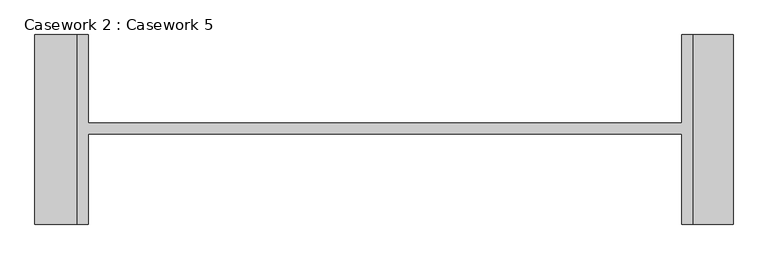
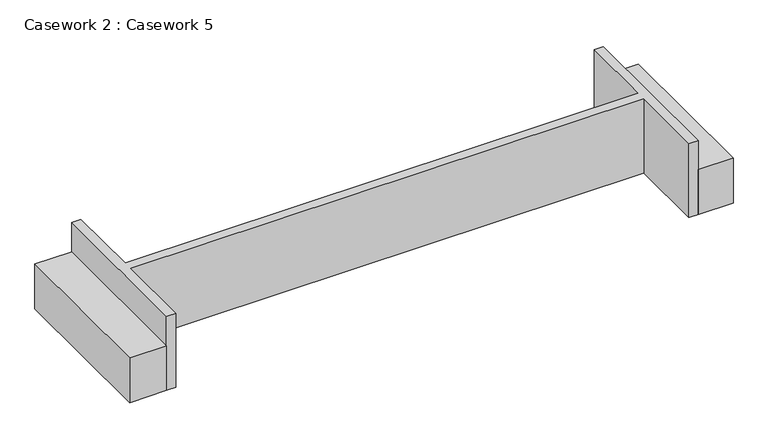
"""IFC4 building model written with IfcOpenShell, lengths in millimetres: furniture geometry, Casework 2 : Casework 5."""

import ifcopenshell
import ifcopenshell.guid

model = None  # the IFC model being written
_history = None  # IfcOwnerHistory: only IFC2X3 demands one
_inside = {}  # id of a spatial element -> (the spatial element, [elements in it])
_under = {}  # id of a project, library or spatial element -> (it, [spatial elements below it])
_declared = {}  # id of a project -> (the project, [libraries it declares])
_typed = {}  # id of a type object -> (the type object, [elements of that type])
_made_of = {}  # id of a material, layer set ... -> (it, [elements and type objects made of it])


def new_model(schema):
    """Start an empty IFC model of exactly this schema.

    Asked for "IFC4X3", IfcOpenShell would pick the latest addendum, in which some entities
    have other attributes; the version numbers below select the first issue.
    IFC2X3 requires an IfcOwnerHistory on every rooted entity: one is made here for all.
    """
    global model, _history
    if schema == "IFC4X3":
        model = ifcopenshell.file(schema_version=(4, 3, 0, 0))
    else:
        model = ifcopenshell.file(schema=schema)
    _inside.clear()
    _under.clear()
    _declared.clear()
    _typed.clear()
    _made_of.clear()
    _history = None
    if model.schema == "IFC2X3":
        org = make("IfcOrganization", Name="unknown")
        user = make(
            "IfcPersonAndOrganization",
            ThePerson=make("IfcPerson", FamilyName="unknown"),
            TheOrganization=org,
        )
        app = make(
            "IfcApplication",
            ApplicationDeveloper=org,
            Version="unknown",
            ApplicationFullName="unknown",
            ApplicationIdentifier="unknown",
        )
        _history = make(
            "IfcOwnerHistory",
            OwningUser=user,
            OwningApplication=app,
            ChangeAction="ADDED",
            CreationDate=0,
        )
    return model


def make(cls, **values):
    """One entity of the class cls with the attributes given. An attribute that is None is left unset."""
    return model.create_entity(
        cls, **{name: value for name, value in values.items() if value is not None}
    )


def rooted(cls, **values):
    """An entity with a GlobalId (a new one), such as an element, a storey or a relation."""
    return make(cls, GlobalId=ifcopenshell.guid.new(), OwnerHistory=_history, **values)


def si_unit(unit_type, name, prefix=None):
    """IfcSIUnit, for example si_unit("LENGTHUNIT", "METRE", prefix="MILLI")."""
    return make("IfcSIUnit", UnitType=unit_type, Prefix=prefix, Name=name)


def assignment(units):
    """IfcUnitAssignment: the units of a project."""
    return None if units is None else make("IfcUnitAssignment", Units=units)


def point(xyz):
    """IfcCartesianPoint."""
    return None if xyz is None else make("IfcCartesianPoint", Coordinates=xyz)


def direction(xyz):
    """IfcDirection."""
    return None if xyz is None else make("IfcDirection", DirectionRatios=xyz)


def frame(location, z_axis=None, x_axis=None):
    """IfcAxis2Placement3D, a coordinate frame: its origin and axes. An axis left out is left unset."""
    return make(
        "IfcAxis2Placement3D",
        Location=point(location),
        Axis=direction(z_axis),
        RefDirection=direction(x_axis),
    )


def origin():
    """The frame at (0, 0, 0) with its axes left unset."""
    return frame((0.0, 0.0, 0.0))


def origin_with_axes():
    """The frame at (0, 0, 0) with the z axis (0, 0, 1) and the x axis (1, 0, 0) written out."""
    return frame((0.0, 0.0, 0.0), z_axis=(0.0, 0.0, 1.0), x_axis=(1.0, 0.0, 0.0))


def place(relative_to, where):
    """IfcLocalPlacement: puts the frame where relative to a parent placement (None: the world)."""
    return make(
        "IfcLocalPlacement", PlacementRelTo=relative_to, RelativePlacement=where
    )


def context(
    kind, dimensions, precision=None, world=None, true_north=None, identifier=None
):
    """IfcGeometricRepresentationContext, for example the 3D "Model" context."""
    return make(
        "IfcGeometricRepresentationContext",
        ContextIdentifier=identifier,
        ContextType=kind,
        CoordinateSpaceDimension=dimensions,
        Precision=precision,
        WorldCoordinateSystem=world,
        TrueNorth=true_north,
    )


def project(units=None, contexts=None):
    """IfcProject with its units and contexts."""
    return rooted(
        "IfcProject",
        Name="project",
        RepresentationContexts=contexts,
        UnitsInContext=assignment(units),
    )


def spatial(cls, under=None, at=None, **own):
    """A site, building, storey or space (cls), placed at a placement, below another one or the project."""
    s = rooted(cls, ObjectPlacement=at, **own)
    if under is not None:
        _under.setdefault(under.id(), (under, []))[1].append(s)
    return s


def polyline(points):
    """IfcPolyline through the points."""
    return make("IfcPolyline", Points=[point(p) for p in points])


def outline(outer, holes=None, kind="AREA"):
    """IfcArbitraryClosedProfileDef: a profile drawn as a closed curve; with holes, ...WithVoids."""
    if holes is None:
        return make("IfcArbitraryClosedProfileDef", ProfileType=kind, OuterCurve=outer)
    return make(
        "IfcArbitraryProfileDefWithVoids",
        ProfileType=kind,
        OuterCurve=outer,
        InnerCurves=holes,
    )


def extrude(swept, where, along, depth):
    """IfcExtrudedAreaSolid: the profile swept, set in the frame where, extruded along a direction by depth."""
    return make(
        "IfcExtrudedAreaSolid",
        SweptArea=swept,
        Position=where,
        ExtrudedDirection=direction(along),
        Depth=depth,
    )


def shape(context_of_items, identifier, shape_type, items):
    """IfcShapeRepresentation: the items that make up one representation, for example the "Body"."""
    return make(
        "IfcShapeRepresentation",
        ContextOfItems=context_of_items,
        RepresentationIdentifier=identifier,
        RepresentationType=shape_type,
        Items=items,
    )


def source(mapping_origin, context_of_items, identifier, shape_type, items):
    """IfcRepresentationMap: a shape defined once, which mapped items show again and again."""
    return make(
        "IfcRepresentationMap",
        MappingOrigin=mapping_origin,
        MappedRepresentation=shape(context_of_items, identifier, shape_type, items),
    )


def transform(
    local_origin,
    x_axis=None,
    y_axis=None,
    z_axis=None,
    scale=None,
    scale2=None,
    scale3=None,
    uniform=True,
):
    """IfcCartesianTransformationOperator3D, or its non-uniform kind. x_axis, y_axis, z_axis: its Axis1, 2, 3."""
    if uniform:
        return make(
            "IfcCartesianTransformationOperator3D",
            Axis1=direction(x_axis),
            Axis2=direction(y_axis),
            LocalOrigin=point(local_origin),
            Scale=scale,
            Axis3=direction(z_axis),
        )
    return make(
        "IfcCartesianTransformationOperator3DnonUniform",
        Axis1=direction(x_axis),
        Axis2=direction(y_axis),
        LocalOrigin=point(local_origin),
        Scale=scale,
        Axis3=direction(z_axis),
        Scale2=scale2,
        Scale3=scale3,
    )


def mapped(mapping_source, mapping_target):
    """IfcMappedItem: shows the shape of a source again, moved by a transform."""
    return make(
        "IfcMappedItem", MappingSource=mapping_source, MappingTarget=mapping_target
    )


def made_of(thing, what):
    """Note that an element or type object is made of a material, layer set ...; save() writes the relation."""
    if what is not None:
        _made_of.setdefault(what.id(), (what, []))[1].append(thing)
    return thing


def element(
    cls,
    number,
    at=None,
    inside=None,
    cuts=None,
    type_object=None,
    material=None,
    context=None,
    identifier="Body",
    shape_type=None,
    held_by="IfcProductDefinitionShape",
    body=None,
    shapes=None,
    **own,
):
    """One element of the class cls, such as IfcWall. Its Tag is "e" and its number.

    at: its placement. inside: the storey or other place that contains it. cuts: it is an
    opening in that element (IfcRelVoidsElement). A single representation is given by context,
    identifier, shape_type and body (its items); several are given by shapes. held_by: the class
    of the entity that holds the representations. save() writes the other relations.
    """
    e = rooted(cls, Tag="e%d" % number, ObjectPlacement=at, **own)
    if body is not None:
        shapes = [shape(context, identifier, shape_type, body)]
    if shapes is not None:
        e.Representation = make(held_by, Representations=shapes)
    if inside is not None:
        _inside.setdefault(inside.id(), (inside, []))[1].append(e)
    if cuts is not None:
        rooted(
            "IfcRelVoidsElement", RelatingBuildingElement=cuts, RelatedOpeningElement=e
        )
    if type_object is not None:
        _typed.setdefault(type_object.id(), (type_object, []))[1].append(e)
    return made_of(e, material)


def aggregate(whole, parts):
    """IfcRelAggregates: a whole, such as a stair, and the parts it consists of."""
    return rooted("IfcRelAggregates", RelatingObject=whole, RelatedObjects=parts)


def save(model, path):
    """Write the relations noted so far, then the file.

    IfcRelAggregates (storeys below a building ...), IfcRelContainedInSpatialStructure (elements
    in a storey), IfcRelDefinesByType, IfcRelAssociatesMaterial and IfcRelDeclares: one each for
    every whole, place, type object, material and project.
    """
    for whole, parts in _under.values():
        aggregate(whole, parts)
    for where, things in _inside.values():
        rooted(
            "IfcRelContainedInSpatialStructure",
            RelatedElements=things,
            RelatingStructure=where,
        )
    for kind, things in _typed.values():
        rooted("IfcRelDefinesByType", RelatedObjects=things, RelatingType=kind)
    for what, things in _made_of.values():
        rooted("IfcRelAssociatesMaterial", RelatedObjects=things, RelatingMaterial=what)
    for by, libraries in _declared.values():
        rooted("IfcRelDeclares", RelatingContext=by, RelatedDefinitions=libraries)
    model.write(path)


def casework_2_casework_5_f543e391(model_context):
    return source(origin(), model_context, "Body", "SweptSolid", [
        extrude(outline(polyline([(-45711.923082, 267678.5135341), (-45711.923082, 265137.4622246), (-46255.3301106, 265137.4622246), (-46255.3301106, 267678.5135341), (-45711.923082, 267678.5135341)])), origin_with_axes(), (0.0, 0.0, 1.0), 736.6),
        extrude(outline(polyline([(-54498.404085, 267678.5135341), (-54498.404085, 265137.4622246), (-55069.0832901, 265137.4622246), (-55069.0832901, 267678.5135341), (-54498.404085, 267678.5135341)])), origin_with_axes(), (0.0, 0.0, 1.0), 736.6),
        extrude(outline(polyline([(-54355.5266335, 267678.5135341), (-54355.5266335, 266491.3050198), (-46397.0475446, 266491.3050198), (-46397.0475446, 267678.5135341), (-46255.3301106, 267678.5135341), (-46255.3301106, 265137.4622246), (-46397.0475446, 265137.4622246), (-46397.0475446, 266349.4417013), (-54355.5266335, 266349.4417013), (-54355.5266335, 265137.4622246), (-54498.404085, 265137.4622246), (-54498.404085, 267678.5135341), (-54355.5266335, 267678.5135341)])), origin_with_axes(), (0.0, 0.0, 1.0), 1219.2),
    ])


if __name__ == "__main__":
    model = new_model("IFC4")
    model_context = context("Model", 3, world=origin())
    ifc_project = project(units=[si_unit("LENGTHUNIT", "METRE", prefix="MILLI")], contexts=[model_context])
    site = spatial("IfcSite", under=ifc_project)
    building = spatial("IfcBuilding", under=site)
    placement = place(None, origin())
    casework_2_casework_5_shape = casework_2_casework_5_f543e391(model_context)
    element("IfcFurniture", 1, ObjectType="Casework 2 : Casework 5", at=placement, inside=building, context=model_context, shape_type="MappedRepresentation", body=[
        mapped(casework_2_casework_5_shape, transform((0.0, 0.0, 0.0), x_axis=(1.0, 0.0, 0.0), y_axis=(0.0, 1.0, 0.0), z_axis=(0.0, 0.0, 1.0))),
    ])
    save(model, "model.ifc")

# Revit data of these elements
# Element 1 (IfcFurniture, "Casework 2 : Casework 5")
#   Materials on its faces: "1.50\" ASPHALT SURFACE COURSE (E-0.3)"
# Materials
#   "1.50\" ASPHALT SURFACE COURSE (E-0.3)": class "Miscellaneous", colour RGB 164 164 164, transparency 0, Cost = 0
